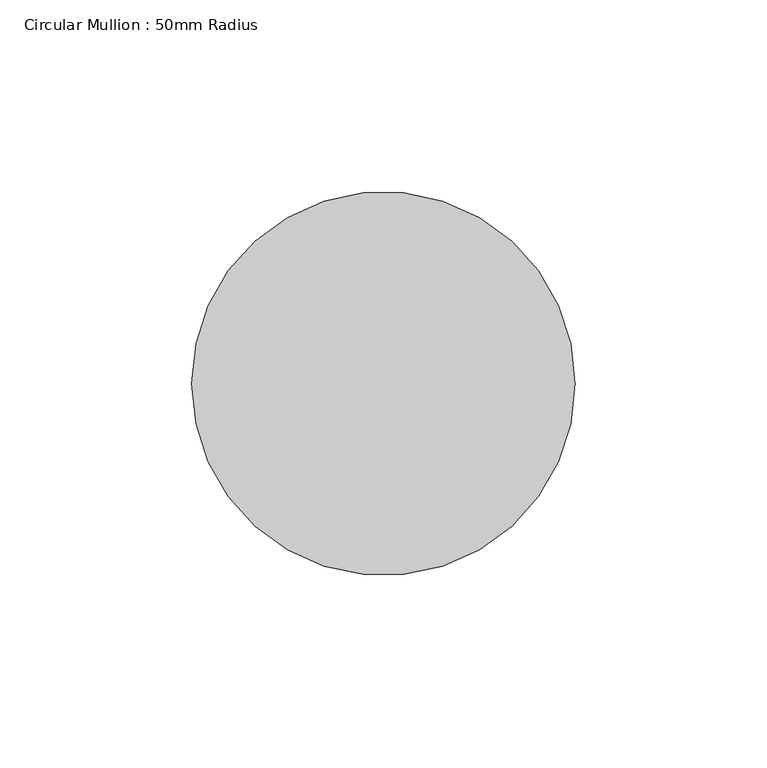
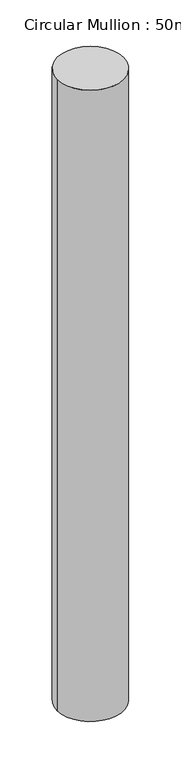
"""IFC4 building model written with IfcOpenShell, lengths in millimetres: member geometry, Circular Mullion : 50mm Radius."""

from ifc_helpers import new_model, si_unit, point, frame, origin, origin_2d, place, context, project, spatial, circle_curve, trimmed, segment, composite_curve, outline, extrude, source, transform, mapped, element, save


def circular_mullion_50mm_radius_460c77b0(model_context):
    return source(origin(), model_context, "Body", "SweptSolid", [
        extrude(outline(composite_curve([segment(trimmed(circle_curve(origin_2d(), 50.0), [point((50.0, 0.0))], [point((-50.0, 0.0))], False, "CARTESIAN"), True, "CONTINUOUS"), segment(trimmed(circle_curve(origin_2d(), 50.0), [point((-50.0, 0.0))], [point((50.0, 0.0))], False, "CARTESIAN"), True, "CONTINUOUS")], self_intersect=False)), frame((0.0, 0.0, -1005.5563843), z_axis=(0.0, 0.0, 1.0), x_axis=(1.0, 0.0, 0.0)), (0.0, 0.0, 1.0), 1005.5563843),
    ])


if __name__ == "__main__":
    model = new_model("IFC4")
    model_context = context("Model", 3, world=origin())
    ifc_project = project(units=[si_unit("LENGTHUNIT", "METRE", prefix="MILLI")], contexts=[model_context])
    site = spatial("IfcSite", under=ifc_project)
    building = spatial("IfcBuilding", under=site)
    placement = place(None, origin())
    circular_mullion_50mm_radius_shape = circular_mullion_50mm_radius_460c77b0(model_context)
    element("IfcMember", 1, ObjectType="Circular Mullion : 50mm Radius", at=placement, inside=building, context=model_context, shape_type="MappedRepresentation", body=[
        mapped(circular_mullion_50mm_radius_shape, transform((0.0, 0.0, 0.0), x_axis=(1.0, 0.0, 0.0), y_axis=(0.0, 1.0, 0.0), z_axis=(0.0, 0.0, 1.0))),
    ])
    save(model, "model.ifc")

# Revit data of these elements
# Type "Circular Mullion : 50mm Radius"
#   built-in parameter 1007350 = 0.164042 (stored number, unit not read)
# Element 1 (IfcMember, "Circular Mullion : 50mm Radius")
#   Materials on its faces: "Aluminium"
# Materials
#   "Aluminium": class "Metal", colour RGB 247 247 247, transparency 0, Description = "Aluminium 6061", Cost = 0
